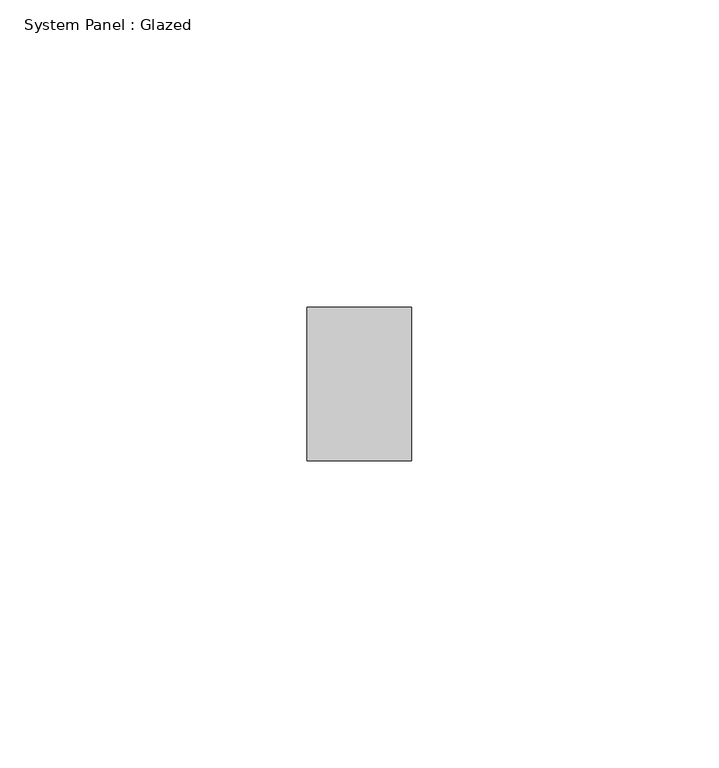
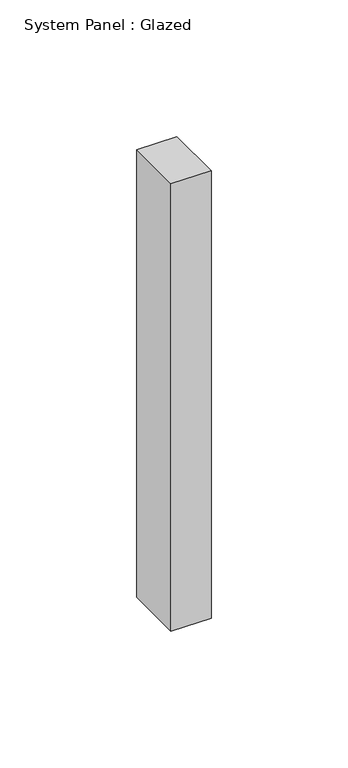
"""IFC4 building model written with IfcOpenShell, lengths in millimetres: plate geometry, System Panel : Glazed."""

from ifc_helpers import new_model, si_unit, origin, origin_with_axes, place, context, project, spatial, polyline, outline, extrude, source, transform, mapped, element, save


def system_panel_glazed_b646d57f(model_context):
    return source(origin(), model_context, "Body", "SweptSolid", [
        extrude(outline(polyline([(8.5363468, 24.5), (-8.5363468, 24.5), (-8.5363468, 49.5), (8.5363468, 49.5), (8.5363468, 24.5)])), origin_with_axes(), (0.0, 0.0, 1.0), 200.0),
    ])


if __name__ == "__main__":
    model = new_model("IFC4")
    model_context = context("Model", 3, world=origin())
    ifc_project = project(units=[si_unit("LENGTHUNIT", "METRE", prefix="MILLI")], contexts=[model_context])
    site = spatial("IfcSite", under=ifc_project)
    building = spatial("IfcBuilding", under=site)
    placement = place(None, origin())
    system_panel_glazed_shape = system_panel_glazed_b646d57f(model_context)
    element("IfcPlate", 1, ObjectType="System Panel : Glazed", at=placement, inside=building, context=model_context, shape_type="MappedRepresentation", body=[
        mapped(system_panel_glazed_shape, transform((0.0, 0.0, 0.0), x_axis=(1.0, 0.0, 0.0), y_axis=(0.0, 1.0, 0.0), z_axis=(0.0, 0.0, 1.0))),
    ])
    save(model, "model.ifc")

# Revit data of these elements
# Element 1 (IfcPlate, "System Panel : Glazed")
#   Materials on its faces: "Glass"
# Materials
#   "Glass": class "Glass", colour RGB 218 227 224, transparency 0.85, Description = "Soda Lime Glass", Cost = 0
